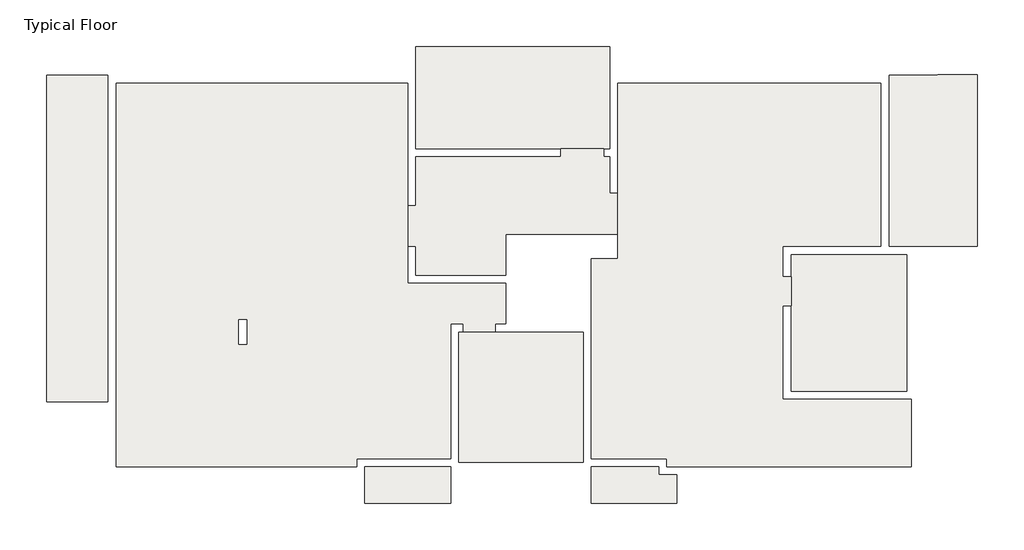
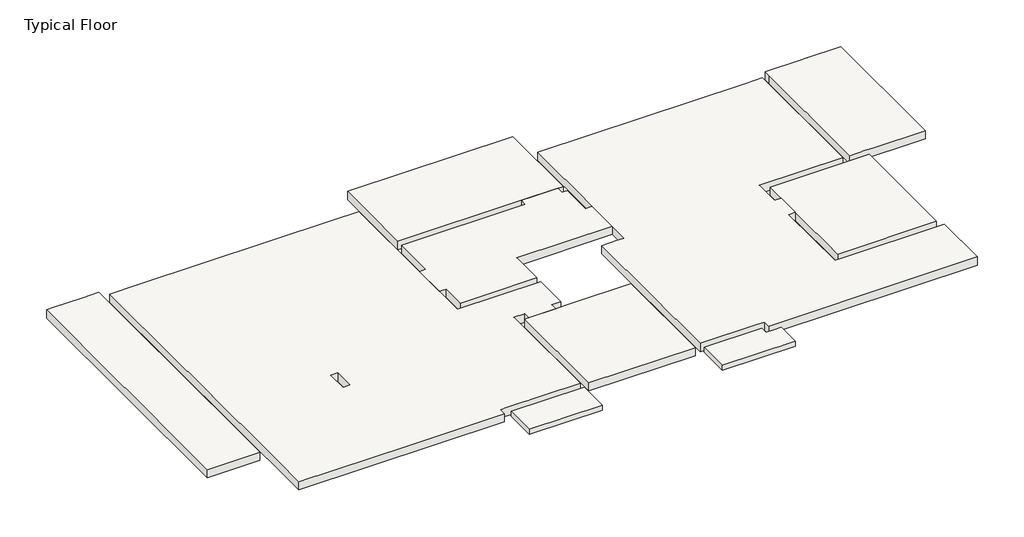
# One storey: 10 slabs.
"""IFC4 building model written with IfcOpenShell, lengths in millimetres."""

from ifc_helpers import new_model, si_unit, origin, place, context, project, spatial, faceted_brep, element, save

model = new_model("IFC4")

# Units and contexts
model_context = context("Model", 3, world=origin())
ifc_project = project(units=[si_unit("LENGTHUNIT", "METRE", prefix="MILLI")], contexts=[model_context])

# Site, building, storey
site = spatial("IfcSite", under=ifc_project)
building = spatial("IfcBuilding", under=site)
storey = spatial("IfcBuildingStorey", under=building, Name="Typical Floor", Elevation=3100.0)

# Slabs
placement = place(None, origin())
element("IfcSlab", 1, ObjectType="15", at=placement, inside=storey, context=model_context, shape_type="Brep", body=[
    faceted_brep([(-43423.3967361, 9899.1553159, 2950.0), (-43423.3967361, 8999.6844165, 2950.0), (-45522.0604135, 8999.6844165, 2950.0), (-45522.0604135, 9899.1553159, 2950.0), (-43423.3967361, 9899.1553159, 3100.0), (-45522.0604135, 9899.1553159, 3100.0), (-45522.0604135, 9699.1553159, 3100.0), (-45522.0604135, 8999.6844165, 3100.0), (-43423.3967361, 8999.6844165, 3100.0)], [[[0, 1, 2, 3]], [[4, 5, 6, 7, 8]], [[1, 0, 4, 8]], [[2, 1, 8, 7]], [[3, 2, 7, 6, 5]], [[0, 3, 5, 4]]]),
])
element("IfcSlab", 2, ObjectType="15", at=placement, inside=storey, context=model_context, shape_type="Brep", body=[
    faceted_brep([(-38322.0604135, 9899.1553159, 2950.0), (-38322.0604135, 9699.1553159, 2950.0), (-38122.0604135, 9699.1553159, 2950.0), (-37873.6612863, 9699.1553159, 2950.0), (-37873.6612863, 8999.1553159, 2950.0), (-39973.6612863, 8999.1553159, 2950.0), (-39973.6612863, 9899.1553159, 2950.0), (-38322.0604135, 9699.1553159, 3100.0), (-38322.0604135, 9899.1553159, 3100.0), (-39973.6612863, 9899.1553159, 3100.0), (-39973.6612863, 8999.6844165, 3100.0), (-39973.6612863, 8999.1553159, 3100.0), (-37873.6612863, 8999.1553159, 3100.0), (-37873.6612863, 9699.1553159, 3100.0), (-38122.0604135, 9699.1553159, 3100.0)], [[[0, 1, 2, 3, 4, 5, 6]], [[7, 8, 9, 10, 11, 12, 13, 14]], [[1, 0, 8, 7]], [[1, 7, 14, 13, 3, 2]], [[4, 3, 13, 12]], [[5, 4, 12, 11]], [[6, 5, 11, 10, 9]], [[0, 6, 9, 8]]]),
])
element("IfcSlab", 3, ObjectType="25", at=placement, inside=storey, context=model_context, shape_type="Brep", body=[
    faceted_brep([(-39522.8676355, 20200.7426175, 2850.0), (-39522.8676355, 17700.213517, 2850.0), (-39672.0739847, 17700.213517, 2850.0), (-40723.9258366, 17700.213517, 2850.0), (-44272.0739847, 17700.213517, 2850.0), (-44272.0739847, 20200.7426175, 2850.0), (-39522.8676355, 20200.7426175, 3100.0), (-44272.0739847, 20200.7426175, 3100.0), (-44272.0739847, 17700.213517, 3100.0), (-40723.9258366, 17700.213517, 3100.0), (-39672.0739847, 17700.213517, 3100.0), (-39522.8676355, 17700.213517, 3100.0)], [[[0, 1, 2, 3, 4, 5]], [[6, 7, 8, 9, 10, 11]], [[1, 0, 6, 11]], [[4, 3, 2, 1, 11, 10, 9, 8]], [[5, 4, 8, 7]], [[0, 5, 7, 6]]]),
])
element("IfcSlab", 4, ObjectType="25", at=placement, inside=storey, context=model_context, shape_type="Brep", body=[
    faceted_brep([(-44472.0739847, 16301.2717181, 2850.0), (-44272.0739847, 16301.2717181, 2850.0), (-44272.0739847, 17500.213517, 2850.0), (-40723.9258366, 17500.213517, 2850.0), (-40723.9258366, 17700.213517, 2850.0), (-39672.0739847, 17700.213517, 2850.0), (-39672.0739847, 17500.213517, 2850.0), (-39522.8676355, 17500.213517, 2850.0), (-39522.8676355, 16599.6844165, 2850.0), (-39322.8676355, 16599.6844165, 2850.0), (-39322.8676355, 15601.2717181, 2850.0), (-42072.0739847, 15601.2717181, 2850.0), (-42072.0739847, 15501.2717181, 2850.0), (-42072.0739847, 14599.6844165, 2850.0), (-44272.0739847, 14599.6844165, 2850.0), (-44272.0739847, 15300.213517, 2850.0), (-44472.0739847, 15300.213517, 2850.0), (-44272.0739847, 16301.2717181, 3100.0), (-44472.0739847, 16301.2717181, 3100.0), (-44472.0739847, 15300.213517, 3100.0), (-44272.0739847, 15300.213517, 3100.0), (-44272.0739847, 14599.6844165, 3100.0), (-42072.0739847, 14599.6844165, 3100.0), (-42072.0739847, 15501.2717181, 3100.0), (-42072.0739847, 15601.2717181, 3100.0), (-39322.8676355, 15601.2717181, 3100.0), (-39322.8676355, 16599.6844165, 3100.0), (-39522.8676355, 16599.6844165, 3100.0), (-39522.8676355, 17500.213517, 3100.0), (-39672.0739847, 17500.213517, 3100.0), (-39672.0739847, 17700.213517, 3100.0), (-40723.9258366, 17700.213517, 3100.0), (-40723.9258366, 17500.213517, 3100.0), (-44272.0739847, 17500.213517, 3100.0)], [[[0, 1, 2, 3, 4, 5, 6, 7, 8, 9, 10, 11, 12, 13, 14, 15, 16]], [[17, 18, 19, 20, 21, 22, 23, 24, 25, 26, 27, 28, 29, 30, 31, 32, 33]], [[1, 0, 18, 17]], [[2, 1, 17, 33]], [[3, 2, 33, 32]], [[4, 3, 32, 31]], [[5, 4, 31, 30]], [[6, 5, 30, 29]], [[7, 6, 29, 28]], [[8, 7, 28, 27]], [[9, 8, 27, 26]], [[10, 9, 26, 25]], [[11, 10, 25, 24]], [[11, 24, 23, 22, 13, 12]], [[14, 13, 22, 21]], [[15, 14, 21, 20]], [[16, 15, 20, 19]], [[0, 16, 19, 18]]]),
])
element("IfcSlab", 5, ObjectType="25", at=placement, inside=storey, context=model_context, shape_type="Brep", body=[
    faceted_brep([(-44472.0739847, 14399.6844165, 2850.0), (-42072.0739847, 14399.6844165, 2850.0), (-42072.0739847, 13399.6844165, 2850.0), (-42328.1586408, 13399.6844165, 2850.0), (-42328.1586408, 13199.6844165, 2850.0), (-43113.343826, 13199.6844165, 2850.0), (-43113.343826, 13399.6844165, 2850.0), (-43423.3967361, 13399.6844165, 2850.0), (-43423.3967361, 13199.6844165, 2850.0), (-43423.3967361, 10099.1553159, 2850.0), (-45522.0604135, 10099.1553159, 2850.0), (-45722.0604135, 10099.1553159, 2850.0), (-45722.0604135, 9899.1553159, 2850.0), (-51622.338535, 9899.1553159, 2850.0), (-51622.338535, 19297.0389138, 2850.0), (-50823.3967361, 19297.0389138, 2850.0), (-50823.3967361, 19300.213517, 2850.0), (-44472.0739847, 19300.213517, 2850.0), (-44472.0739847, 16301.2717181, 2850.0), (-44472.0739847, 15300.213517, 2850.0), (-44472.0739847, 14599.6844165, 2850.0), (-48420.2494744, 13497.0617054, 2850.0), (-48620.2494744, 13497.0617054, 2850.0), (-48620.2494744, 12897.0617054, 2850.0), (-48420.2494744, 12897.0617054, 2850.0), (-42072.0739847, 14399.6844165, 3100.0), (-44472.0739847, 14399.6844165, 3100.0), (-44472.0739847, 14599.6844165, 3100.0), (-44472.0739847, 15300.213517, 3100.0), (-44472.0739847, 16301.2717181, 3100.0), (-44472.0739847, 19300.213517, 3100.0), (-45172.6030853, 19300.213517, 3100.0), (-50823.3967361, 19300.213517, 3100.0), (-50823.3967361, 19297.0389138, 3100.0), (-51622.338535, 19297.0389138, 3100.0), (-51622.338535, 18701.2717181, 3100.0), (-51622.338535, 14321.5649818, 3100.0), (-51622.338535, 13521.5649818, 3100.0), (-51622.338535, 12125.6103424, 3100.0), (-51622.338535, 9899.1553159, 3100.0), (-48522.8676355, 9899.1553159, 3100.0), (-45722.0604135, 9899.1553159, 3100.0), (-45722.0604135, 10099.1553159, 3100.0), (-45522.0604135, 10099.1553159, 3100.0), (-43423.3967361, 10099.1553159, 3100.0), (-43423.3967361, 13199.6844165, 3100.0), (-43423.3967361, 13399.6844165, 3100.0), (-43113.343826, 13399.6844165, 3100.0), (-43113.343826, 13199.6844165, 3100.0), (-42328.1586408, 13199.6844165, 3100.0), (-42328.1586408, 13399.6844165, 3100.0), (-42072.0739847, 13399.6844165, 3100.0), (-48620.2494744, 13497.0617054, 3100.0), (-48420.2494744, 13497.0617054, 3100.0), (-48420.2494744, 12897.0617054, 3100.0), (-48620.2494744, 12897.0617054, 3100.0)], [[[0, 1, 2, 3, 4, 5, 6, 7, 8, 9, 10, 11, 12, 13, 14, 15, 16, 17, 18, 19, 20], [21, 22, 23, 24]], [[25, 26, 27, 28, 29, 30, 31, 32, 33, 34, 35, 36, 37, 38, 39, 40, 41, 42, 43, 44, 45, 46, 47, 48, 49, 50, 51], [52, 53, 54, 55]], [[26, 0, 20, 19, 18, 17, 30, 29, 28, 27]], [[1, 0, 26, 25]], [[2, 1, 25, 51]], [[3, 2, 51, 50]], [[4, 3, 50, 49]], [[5, 4, 49, 48]], [[6, 5, 48, 47]], [[7, 6, 47, 46]], [[7, 46, 45, 44, 9, 8]], [[9, 44, 43, 42, 11, 10]], [[12, 11, 42, 41]], [[13, 12, 41, 40, 39]], [[13, 39, 38, 37, 36, 35, 34, 14]], [[30, 17, 16, 32, 31]], [[22, 21, 53, 52]], [[23, 22, 52, 55]], [[24, 23, 55, 54]], [[21, 24, 54, 53]], [[33, 15, 14, 34]], [[15, 33, 32, 16]]]),
])
element("IfcSlab", 6, ObjectType="25", at=placement, inside=storey, context=model_context, shape_type="Brep", body=[
    faceted_brep([(-40173.6612863, 13199.6844165, 2850.0), (-40173.6612863, 10009.208226, 2850.0), (-43223.3967361, 10009.208226, 2850.0), (-43223.3967361, 13199.6844165, 2850.0), (-43113.343826, 13199.6844165, 2850.0), (-42328.1586408, 13199.6844165, 2850.0), (-40173.6612863, 10009.208226, 3100.0), (-40173.6612863, 13199.6844165, 3100.0), (-41872.0739847, 13199.6844165, 3100.0), (-42328.1586408, 13199.6844165, 3100.0), (-43113.343826, 13199.6844165, 3100.0), (-43223.3967361, 13199.6844165, 3100.0), (-43223.3967361, 10009.208226, 3100.0)], [[[0, 1, 2, 3, 4, 5]], [[6, 7, 8, 9, 10, 11, 12]], [[1, 0, 7, 6]], [[2, 1, 6, 12]], [[3, 2, 12, 11]], [[3, 11, 10, 9, 8, 7, 0, 5, 4]]]),
])
element("IfcSlab", 7, ObjectType="25", at=placement, inside=storey, context=model_context, shape_type="Brep", body=[
    faceted_brep([(-32233.9258366, 15100.213517, 2850.0), (-32233.9258366, 11749.9489667, 2850.0), (-35074.1903869, 11749.9489667, 2850.0), (-35074.1903869, 13846.245263, 2850.0), (-35074.1903869, 14551.0071678, 2850.0), (-35074.1903869, 15100.213517, 2850.0), (-32233.9258366, 15100.213517, 3100.0), (-35074.1903869, 15100.213517, 3100.0), (-35074.1903869, 14551.0071678, 3100.0), (-35074.1903869, 13846.245263, 3100.0), (-35074.1903869, 11749.9489667, 3100.0), (-32233.9258366, 11749.9489667, 3100.0)], [[[0, 1, 2, 3, 4, 5]], [[6, 7, 8, 9, 10, 11]], [[1, 0, 6, 11]], [[2, 1, 11, 10]], [[5, 4, 3, 2, 10, 9, 8, 7]], [[0, 5, 7, 6]]]),
])
element("IfcSlab", 8, ObjectType="25", at=placement, inside=storey, context=model_context, shape_type="Brep", body=[
    faceted_brep([(-32874.1903869, 15300.213517, 2850.0), (-35274.1903869, 15300.213517, 2850.0), (-35274.1903869, 15100.213517, 2850.0), (-35274.1903869, 14551.0071678, 2850.0), (-35074.1903869, 14551.0071678, 2850.0), (-35074.1903869, 13846.245263, 2850.0), (-35274.1903869, 13846.245263, 2850.0), (-35274.1903869, 11549.9489667, 2850.0), (-35074.1903869, 11549.9489667, 2850.0), (-32123.9258366, 11549.9489667, 2850.0), (-32123.9258366, 9899.1553159, 2850.0), (-38122.0604135, 9899.1553159, 2850.0), (-38122.0604135, 10099.1553159, 2850.0), (-38322.0604135, 10099.1553159, 2850.0), (-39973.6612863, 10099.1553159, 2850.0), (-39973.6612863, 14999.6844165, 2850.0), (-39522.8676355, 14999.6844165, 2850.0), (-39322.8676355, 14999.6844165, 2850.0), (-39322.8676355, 15600.7426175, 2850.0), (-39322.8676355, 15601.2717181, 2850.0), (-39322.8676355, 16599.6844165, 2850.0), (-39322.8676355, 19301.2717181, 2850.0), (-32874.1903869, 19301.2717181, 2850.0), (-32874.1903869, 15700.213517, 2850.0), (-35274.1903869, 15300.213517, 3100.0), (-32874.1903869, 15300.213517, 3100.0), (-32874.1903869, 15700.213517, 3100.0), (-32874.1903869, 19301.2717181, 3100.0), (-33373.6612863, 19301.2717181, 3100.0), (-39322.8676355, 19301.2717181, 3100.0), (-39322.8676355, 16599.6844165, 3100.0), (-39322.8676355, 15601.2717181, 3100.0), (-39322.8676355, 15600.7426175, 3100.0), (-39322.8676355, 14999.6844165, 3100.0), (-39522.8676355, 14999.6844165, 3100.0), (-39973.6612863, 14999.6844165, 3100.0), (-39973.6612863, 10099.1553159, 3100.0), (-38322.0604135, 10099.1553159, 3100.0), (-38122.0604135, 10099.1553159, 3100.0), (-38122.0604135, 9899.1553159, 3100.0), (-32123.9258366, 9899.1553159, 3100.0), (-32123.9258366, 11549.9489667, 3100.0), (-35074.1903869, 11549.9489667, 3100.0), (-35274.1903869, 11549.9489667, 3100.0), (-35274.1903869, 13846.245263, 3100.0), (-35074.1903869, 13846.245263, 3100.0), (-35074.1903869, 14551.0071678, 3100.0), (-35274.1903869, 14551.0071678, 3100.0), (-35274.1903869, 15100.213517, 3100.0)], [[[0, 1, 2, 3, 4, 5, 6, 7, 8, 9, 10, 11, 12, 13, 14, 15, 16, 17, 18, 19, 20, 21, 22, 23]], [[24, 25, 26, 27, 28, 29, 30, 31, 32, 33, 34, 35, 36, 37, 38, 39, 40, 41, 42, 43, 44, 45, 46, 47, 48]], [[25, 0, 23, 22, 27, 26]], [[1, 0, 25, 24]], [[1, 24, 48, 47, 3, 2]], [[4, 3, 47, 46]], [[5, 4, 46, 45]], [[6, 5, 45, 44]], [[7, 6, 44, 43]], [[7, 43, 42, 41, 9, 8]], [[10, 9, 41, 40]], [[11, 10, 40, 39]], [[12, 11, 39, 38]], [[12, 38, 37, 36, 14, 13]], [[15, 14, 36, 35]], [[15, 35, 34, 33, 17, 16]], [[17, 33, 32, 31, 30, 29, 21, 20, 19, 18]], [[22, 21, 29, 28, 27]]]),
])
element("IfcSlab", 9, ObjectType="25", at=placement, inside=storey, context=model_context, shape_type="Brep", body=[
    faceted_brep([(-30505.8186523, 19506.2717181, 2850.0), (-30505.8186523, 15300.213517, 2850.0), (-32674.1903869, 15300.213517, 2850.0), (-32674.1903869, 19301.2717181, 2850.0), (-32673.1321858, 19301.2717181, 2850.0), (-32673.1321858, 19501.2717181, 2850.0), (-31473.1321858, 19501.2717181, 2850.0), (-31473.1321858, 19506.2717181, 2850.0), (-30505.8186523, 15300.213517, 3100.0), (-30505.8186523, 15500.213517, 3100.0), (-30505.8186523, 19501.2717181, 3100.0), (-30505.8186523, 19506.2717181, 3100.0), (-31473.1321858, 19506.2717181, 3100.0), (-31473.1321858, 19501.2717181, 3100.0), (-31665.8186523, 19501.2717181, 3100.0), (-32673.1321858, 19501.2717181, 3100.0), (-32673.1321858, 19301.2717181, 3100.0), (-32674.1903869, 19301.2717181, 3100.0), (-32674.1903869, 15700.213517, 3100.0), (-32674.1903869, 15300.213517, 3100.0), (-32233.9258366, 15300.213517, 3100.0), (-32023.9258366, 15300.213517, 3100.0)], [[[0, 1, 2, 3, 4, 5, 6, 7]], [[8, 9, 10, 11, 12, 13, 14, 15, 16, 17, 18, 19, 20, 21]], [[11, 0, 7, 12]], [[1, 0, 11, 10, 9, 8]], [[2, 1, 8, 21, 20, 19]], [[2, 19, 18, 17, 3]], [[16, 4, 3, 17]], [[4, 16, 15, 5]], [[13, 6, 5, 15, 14]], [[6, 13, 12, 7]]]),
])
element("IfcSlab", 10, ObjectType="25", at=placement, inside=storey, context=model_context, shape_type="Brep", body=[
    faceted_brep([(-51822.338535, 19497.0389138, 2850.0), (-51822.338535, 11493.9394503, 2850.0), (-53328.1898421, 11493.9394503, 2850.0), (-53328.1898421, 19497.0389138, 2850.0), (-51822.338535, 19497.0389138, 3100.0), (-52321.8094345, 19497.0389138, 3100.0), (-53128.1898421, 19497.0389138, 3100.0), (-53328.1898421, 19497.0389138, 3100.0), (-53328.1898421, 11693.9394503, 3100.0), (-53328.1898421, 11493.9394503, 3100.0), (-51822.338535, 11493.9394503, 3100.0), (-51822.338535, 11693.9394503, 3100.0), (-51822.338535, 12125.6103424, 3100.0), (-51822.338535, 13521.5649818, 3100.0), (-51822.338535, 14321.5649818, 3100.0), (-51822.338535, 18701.2717181, 3100.0), (-51822.338535, 19297.0389138, 3100.0)], [[[0, 1, 2, 3]], [[4, 5, 6, 7, 8, 9, 10, 11, 12, 13, 14, 15, 16]], [[1, 0, 4, 16, 15, 14, 13, 12, 11, 10]], [[2, 1, 10, 9]], [[3, 2, 9, 8, 7]], [[0, 3, 7, 6, 5, 4]]]),
])

save(model, "model.ifc")

# Revit data of these elements
# Type "15"
#   Function = 0
#   Layers, outside or top first: 15 cm "Concrete" (function 1)
# Type "25"
#   Function = 0
#   Layers, outside or top first: 25 cm "Concrete" (function 1)
# Element 1 (IfcSlab, "15")
#   Mark = "F9"
#   SOFiSTiK_AMG_Comments = ""
#   Height Offset From Level = 0 cm
#   built-in parameter 1001954 = 1
#   SOFiSTiK_AMG_Scheduled = yes
#   SOFiSTiK_AMG_Adjusted = yes
#   Phase Created = New Construction
#   Materials on its faces: "Concrete"
# Element 2 (IfcSlab, "15")
#   Mark = "F10"
#   SOFiSTiK_AMG_Comments = ""
#   Height Offset From Level = 0 cm
#   built-in parameter 1001954 = 1
#   SOFiSTiK_AMG_Scheduled = yes
#   SOFiSTiK_AMG_Adjusted = yes
#   Phase Created = New Construction
#   Materials on its faces: "Concrete"
# Element 3 (IfcSlab, "25")
#   Mark = "F1"
#   SOFiSTiK_AMG_Comments = ""
#   Height Offset From Level = 0 cm
#   built-in parameter 1001954 = 1
#   SOFiSTiK_AMG_Scheduled = yes
#   SOFiSTiK_AMG_Adjusted = yes
#   Phase Created = New Construction
#   Materials on its faces: "Concrete"
# Element 4 (IfcSlab, "25")
#   Mark = "F2"
#   SOFiSTiK_AMG_Comments = ""
#   built-in parameter 1001955 = 1.5708 (stored number, unit not read)
#   Height Offset From Level = 0 cm
#   built-in parameter 1001954 = 1
#   SOFiSTiK_AMG_Scheduled = yes
#   SOFiSTiK_AMG_Adjusted = yes
#   Phase Created = New Construction
#   Materials on its faces: "Concrete"
# Element 5 (IfcSlab, "25")
#   Mark = "F3"
#   SOFiSTiK_AMG_Comments = ""
#   Height Offset From Level = 0 cm
#   built-in parameter 1001954 = 1
#   SOFiSTiK_AMG_Scheduled = yes
#   SOFiSTiK_AMG_Adjusted = yes
#   Phase Created = New Construction
#   Materials on its faces: "Concrete"
# Element 6 (IfcSlab, "25")
#   Mark = "F4"
#   SOFiSTiK_AMG_Comments = ""
#   Height Offset From Level = 0 cm
#   built-in parameter 1001954 = 1
#   SOFiSTiK_AMG_Scheduled = yes
#   SOFiSTiK_AMG_Adjusted = yes
#   Phase Created = New Construction
#   Materials on its faces: "Concrete"
# Element 7 (IfcSlab, "25")
#   Mark = "F5"
#   SOFiSTiK_AMG_Comments = ""
#   Height Offset From Level = 0 cm
#   built-in parameter 1001954 = 1
#   SOFiSTiK_AMG_Scheduled = yes
#   SOFiSTiK_AMG_Adjusted = yes
#   Phase Created = New Construction
#   Materials on its faces: "Concrete"
# Element 8 (IfcSlab, "25")
#   Mark = "F6"
#   SOFiSTiK_AMG_Comments = ""
#   Height Offset From Level = 0 cm
#   built-in parameter 1001954 = 1
#   SOFiSTiK_AMG_Scheduled = yes
#   SOFiSTiK_AMG_Adjusted = yes
#   Phase Created = New Construction
#   Materials on its faces: "Concrete"
# Element 9 (IfcSlab, "25")
#   Mark = "F7"
#   SOFiSTiK_AMG_Comments = ""
#   built-in parameter 1001955 = 3.14159 (stored number, unit not read)
#   Height Offset From Level = 0 cm
#   built-in parameter 1001954 = 1
#   SOFiSTiK_AMG_Scheduled = yes
#   SOFiSTiK_AMG_Adjusted = yes
#   Phase Created = New Construction
#   Materials on its faces: "Concrete"
# Element 10 (IfcSlab, "25")
#   Mark = "F8"
#   SOFiSTiK_AMG_Comments = ""
#   Height Offset From Level = 0 cm
#   built-in parameter 1001954 = 1
#   SOFiSTiK_AMG_Scheduled = yes
#   SOFiSTiK_AMG_Adjusted = yes
#   Phase Created = New Construction
#   Materials on its faces: "Concrete"
# Materials
#   "Concrete": class "Concrete", colour RGB 192 192 192, transparency 0, Keynote = "01000", Description = "Cast-in-place concrete", Cost = 0
